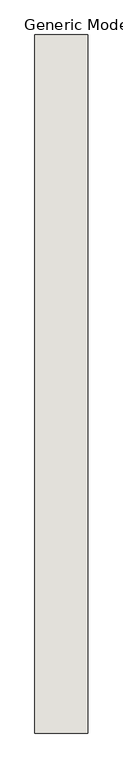
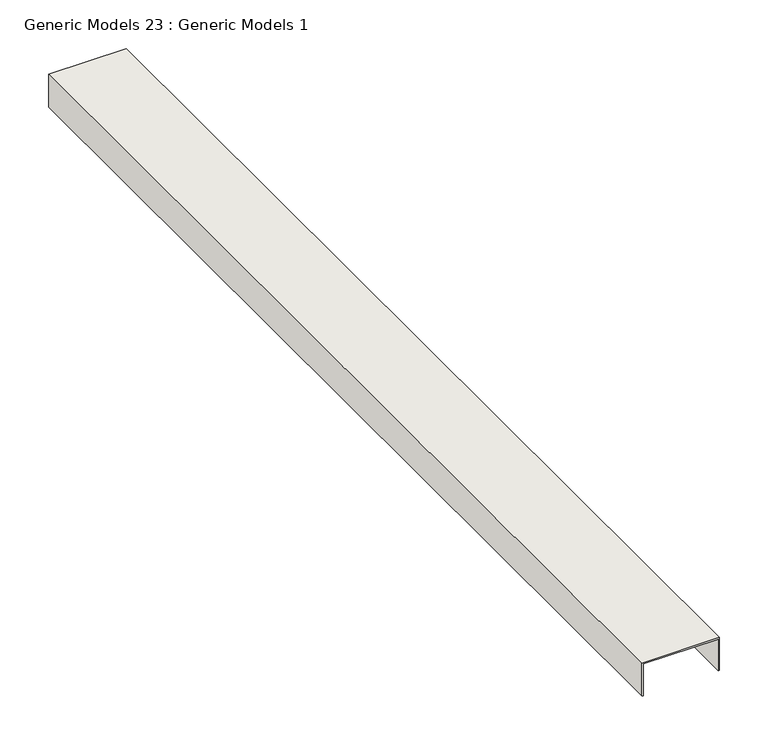
"""IFC4 building model written with IfcOpenShell, lengths in millimetres: wall geometry, Generic Models 23 : Generic Models 1."""

from ifc_helpers import new_model, si_unit, frame, origin, place, context, project, spatial, polyline, outline, extrude, source, transform, mapped, element, save


def generic_models_23_generic_models_1_d2f1e0fb(model_context):
    return source(origin(), model_context, "Body", "SweptSolid", [
        extrude(outline(polyline([(2457.45, 49784.0), (2457.45, 49691.925), (2416.175, 49691.925), (2416.175, 49693.5125), (2455.8625, 49693.5125), (2455.8625, 49782.4125), (2416.175, 49782.4125), (2416.175, 49784.0), (2457.45, 49784.0)])), frame((0.0, 0.0, 0.0), z_axis=(0.0, 1.0, 0.0), x_axis=(0.0, 0.0, 1.0)), (0.0, 0.0, 1.0), 1219.2),
    ])


if __name__ == "__main__":
    model = new_model("IFC4")
    model_context = context("Model", 3, world=origin())
    ifc_project = project(units=[si_unit("LENGTHUNIT", "METRE", prefix="MILLI")], contexts=[model_context])
    site = spatial("IfcSite", under=ifc_project)
    building = spatial("IfcBuilding", under=site)
    placement = place(None, origin())
    generic_models_23_generic_models_1_shape = generic_models_23_generic_models_1_d2f1e0fb(model_context)
    element("IfcWall", 1, ObjectType="Generic Models 23 : Generic Models 1", at=placement, inside=building, context=model_context, shape_type="MappedRepresentation", body=[
        mapped(generic_models_23_generic_models_1_shape, transform((0.0, 0.0, 0.0), x_axis=(1.0, 0.0, 0.0), y_axis=(0.0, 1.0, 0.0), z_axis=(0.0, 0.0, 1.0))),
    ])
    save(model, "model.ifc")

# Revit data of these elements
# Element 1 (IfcWall, "Generic Models 23 : Generic Models 1")
#   Materials on its faces: "DEEP LEG OF DEFLECTION TRACK (2\" MIN. DEFLECTION)"
# Materials
#   "DEEP LEG OF DEFLECTION TRACK (2\" MIN. DEFLECTION)": class "Unassigned", colour RGB 210 209 208, transparency 0, Keynote = "M05121300.02", Cost = 0
